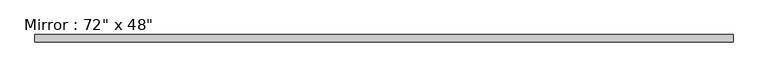
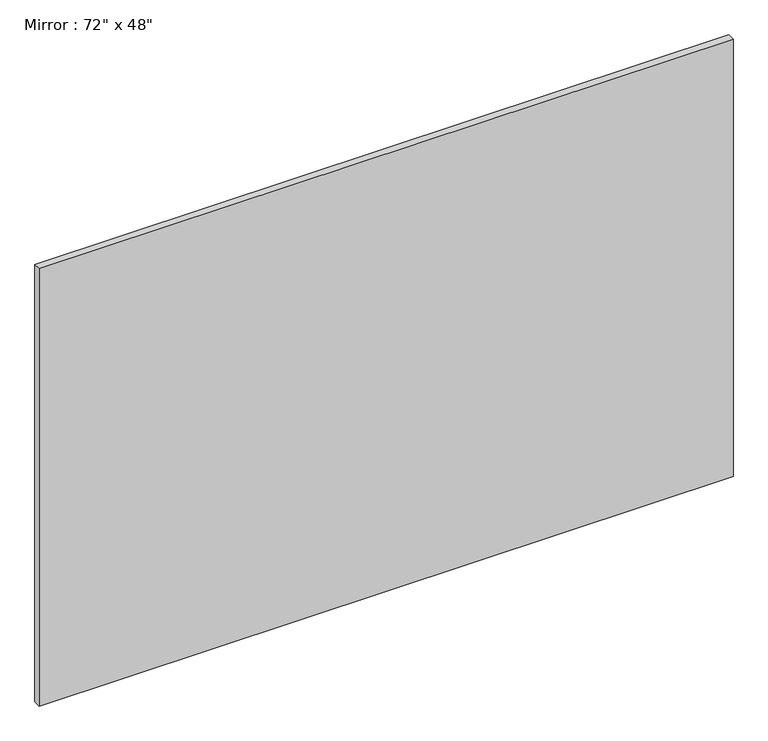
"""IFC4 building model written with IfcOpenShell, lengths in millimetres: proxy geometry."""

from ifc_helpers import new_model, si_unit, frame, origin, place, context, project, spatial, polyline, outline, extrude, source, transform, mapped, element, save


def proxy_e7df19ba(model_context):
    return source(origin(), model_context, "Body", "SweptSolid", [
        extrude(outline(polyline([(-889.9296989, -82.55), (-889.9296989, -63.5), (938.8703011, -63.5), (938.8703011, -82.55), (-889.9296989, -82.55)])), frame((0.0, 0.0, 1066.8), z_axis=(0.0, 0.0, 1.0), x_axis=(1.0, 0.0, 0.0)), (0.0, 0.0, 1.0), 1219.2),
    ])


if __name__ == "__main__":
    model = new_model("IFC4")
    model_context = context("Model", 3, world=origin())
    ifc_project = project(units=[si_unit("LENGTHUNIT", "METRE", prefix="MILLI")], contexts=[model_context])
    site = spatial("IfcSite", under=ifc_project)
    building = spatial("IfcBuilding", under=site)
    placement = place(None, origin())
    proxy_shape = proxy_e7df19ba(model_context)
    element("IfcBuildingElementProxy", 1, Name="Mirror : 72\" x 48\"", ObjectType="Mirror : 72\" x 48\"", at=placement, inside=building, context=model_context, shape_type="MappedRepresentation", body=[
        mapped(proxy_shape, transform((0.0, 0.0, 0.0), x_axis=(1.0, 0.0, 0.0), y_axis=(0.0, 1.0, 0.0), z_axis=(0.0, 0.0, 1.0))),
    ])
    save(model, "model.ifc")

# Revit data of these elements
# Type "Mirror : 72\" x 48\""
#   Assembly Code = "C1030200"
#   Height = 4' - 0"
#   Mounting Height = 3' - 6"
#   Width = 6' - 0"
#   Default Elevation = 0
# Element 1 (IfcBuildingElementProxy, "Mirror : 72\" x 48\"")
#   Materials on its faces: "Mirror"
# Materials
#   "Mirror": class "Glass", colour RGB 120 120 120, transparency 0, Description = "Mirror glass", Cost = 0
